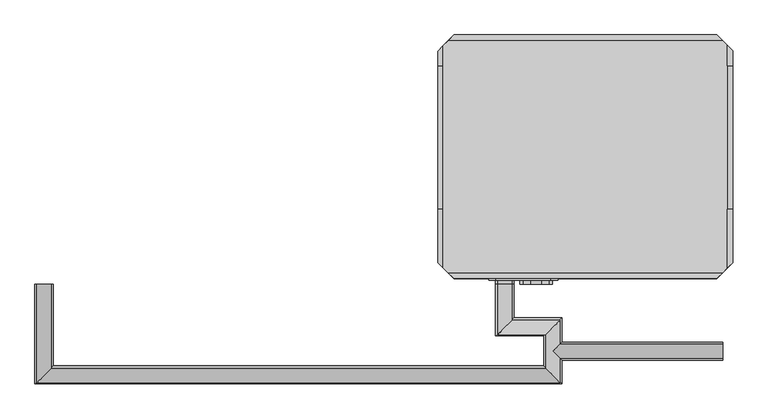
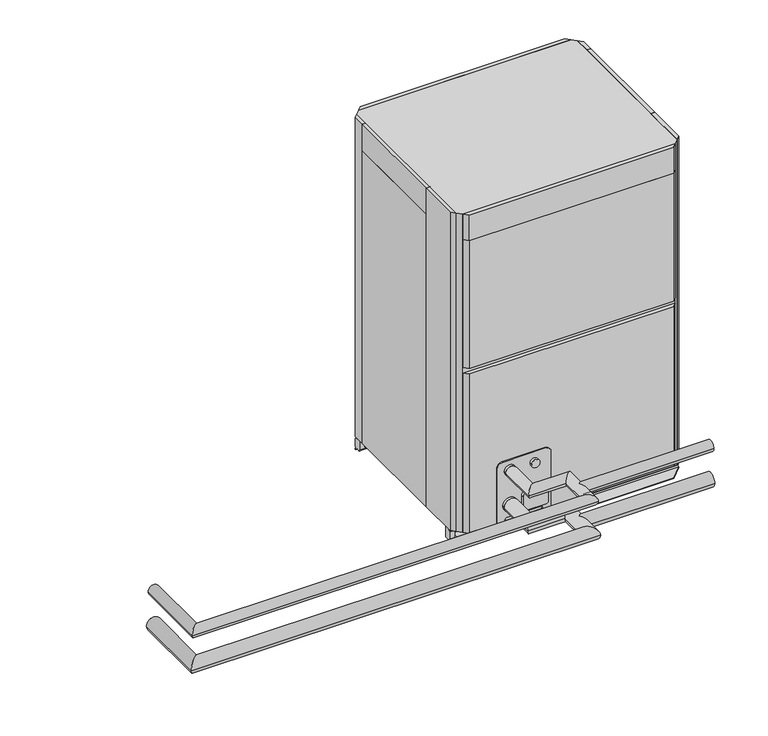
"""IFC4 building model written with IfcOpenShell, lengths in millimetres: proxy geometry, PURY-P168-288_YSJMU_Heat_Recovery_460V : PURY-P192YSJMU-A(-BS)_460V."""

from ifc_helpers import new_model, si_unit, point, frame, frame_2d, origin, place, context, project, spatial, polyline, circle_curve, ellipse_curve, trimmed, segment, composite_curve, outline, extrude, source, transform, mapped, element, save
from ifc_brep_helpers import plane_surface, cylinder_surface, revolved_surface, advanced_brep


def mechanical_equipment_f1262ded(model_context):
    return source(origin(), model_context, "Body", "SolidModel", [
        advanced_brep(
        [(-227.9552757, -397.2710787, 128.75), (-170.8052757, -397.2710787, 128.75), (-227.9552757, -709.2315266, 128.75), (-170.8052757, -652.0815266, 128.75), (1418.1947243, -709.2315266, 128.75), (1361.0447243, -652.0815266, 128.75), (1418.1947243, -635.3498061, 128.75), (1389.6197243, -606.7748061, 157.325), (1418.1947243, -578.1998061, 128.75), (1418.1947243, -502.0815266, 128.75), (1361.0447243, -559.2315266, 128.75), (1389.6197243, -606.7748061, 100.175), (1268.1947243, -502.0815266, 128.75), (1211.0447243, -559.2315266, 128.75), (1268.1947243, -397.2710787, 128.75), (1211.0447243, -397.2710787, 128.75), (1919.6197243, -635.3498061, 128.75), (1919.6197243, -578.1998061, 128.75)],
        [
            (0, 1, circle_curve(frame((-199.3802757, -397.2710787, 128.75), z_axis=(0.0, 1.0, 0.0), x_axis=(1.0, 0.0, 0.0)), 28.575)),
            (1, 0, circle_curve(frame((-199.3802757, -397.2710787, 128.75), z_axis=(0.0, 1.0, 0.0), x_axis=(1.0, 0.0, 0.0)), 28.575)),
            (0, 2),
            (2, 3, ellipse_curve(frame((-199.3802757, -680.6565266, 128.75), z_axis=(-0.7071067811865475, 0.7071067811865475, 0.0), x_axis=(0.7071067811865474, 0.7071067811865476, 0.0)), 40.4111525, 28.575)),
            (3, 1),
            (3, 2, ellipse_curve(frame((-199.3802757, -680.6565266, 128.75), z_axis=(-0.7071067811865475, 0.7071067811865475, 0.0), x_axis=(0.7071067811865474, 0.7071067811865476, 0.0)), 40.4111525, 28.575)),
            (2, 4),
            (4, 5, ellipse_curve(frame((1389.6197243, -680.6565266, 128.75), z_axis=(-0.7071067811865475, -0.7071067811865475, 0.0), x_axis=(-0.7071067811865476, 0.7071067811865474, 0.0)), 40.4111525, 28.575)),
            (5, 3),
            (5, 4, ellipse_curve(frame((1389.6197243, -680.6565266, 128.75), z_axis=(-0.7071067811865475, -0.7071067811865475, 0.0), x_axis=(-0.7071067811865476, 0.7071067811865474, 0.0)), 40.4111525, 28.575)),
            (4, 6),
            (6, 7, ellipse_curve(frame((1389.6197243, -606.7748061, 128.75), z_axis=(-0.7071067811865475, -0.7071067811865475, 0.0), x_axis=(0.7071067811865474, -0.7071067811865476, 0.0)), 40.4111525, 28.575)),
            (7, 8, ellipse_curve(frame((1389.6197243, -606.7748061, 128.75), z_axis=(-0.7071067811865475, 0.7071067811865475, 0.0), x_axis=(-0.7071067811865474, -0.7071067811865476, 0.0)), 40.4111525, 28.575)),
            (8, 9),
            (9, 10, ellipse_curve(frame((1389.6197243, -530.6565266, 128.75), z_axis=(0.7071067811865475, -0.7071067811865475, 0.0), x_axis=(-0.7071067811865474, -0.7071067811865476, 0.0)), 40.4111525, 28.575)),
            (10, 5),
            (10, 9, ellipse_curve(frame((1389.6197243, -530.6565266, 128.75), z_axis=(0.7071067811865475, -0.7071067811865475, 0.0), x_axis=(-0.7071067811865474, -0.7071067811865476, 0.0)), 40.4111525, 28.575)),
            (8, 11, ellipse_curve(frame((1389.6197243, -606.7748061, 128.75), z_axis=(-0.7071067811865475, 0.7071067811865475, 0.0), x_axis=(-0.7071067811865474, -0.7071067811865476, 0.0)), 40.4111525, 28.575)),
            (11, 6, ellipse_curve(frame((1389.6197243, -606.7748061, 128.75), z_axis=(-0.7071067811865475, -0.7071067811865475, 0.0), x_axis=(0.7071067811865474, -0.7071067811865476, 0.0)), 40.4111525, 28.575)),
            (9, 12),
            (12, 13, ellipse_curve(frame((1239.6197243, -530.6565266, 128.75), z_axis=(0.7071067811865475, -0.7071067811865475, 0.0), x_axis=(0.7071067811865476, 0.7071067811865474, 0.0)), 40.4111525, 28.575)),
            (13, 10),
            (13, 12, ellipse_curve(frame((1239.6197243, -530.6565266, 128.75), z_axis=(0.7071067811865475, -0.7071067811865475, 0.0), x_axis=(0.7071067811865476, 0.7071067811865474, 0.0)), 40.4111525, 28.575)),
            (14, 15, circle_curve(frame((1239.6197243, -397.2710787, 128.75), z_axis=(0.0, 1.0, 0.0), x_axis=(-1.0, 0.0, 0.0)), 28.575)),
            (15, 14, circle_curve(frame((1239.6197243, -397.2710787, 128.75), z_axis=(0.0, 1.0, 0.0), x_axis=(-1.0, 0.0, 0.0)), 28.575)),
            (12, 14),
            (15, 13),
            (16, 17, circle_curve(frame((1919.6197243, -606.7748061, 128.75), z_axis=(1.0, 0.0, 0.0), x_axis=(0.0, 1.0, 0.0)), 28.575)),
            (17, 16, circle_curve(frame((1919.6197243, -606.7748061, 128.75), z_axis=(1.0, 0.0, 0.0), x_axis=(0.0, 1.0, 0.0)), 28.575)),
            (17, 8),
            (6, 16),
        ],
        [
            plane_surface(frame((-199.3802757, -397.2710787, 128.75), z_axis=(0.0, 1.0, 0.0), x_axis=(0.0, 0.0, 1.0))),
            cylinder_surface(frame((-199.3802757, -397.2710787, 128.75), z_axis=(0.0, 1.0, 0.0), x_axis=(1.0, 0.0, 0.0)), 28.575),
            cylinder_surface(frame((-199.3802757, -680.6565266, 128.75), z_axis=(-1.0, 0.0, 0.0), x_axis=(0.0, 1.0, 0.0)), 28.575),
            cylinder_surface(frame((1389.6197243, -680.6565266, 128.75), z_axis=(0.0, -1.0, 0.0), x_axis=(-1.0, 0.0, 0.0)), 28.575),
            cylinder_surface(frame((1389.6197243, -530.6565266, 128.75), z_axis=(1.0, 0.0, 0.0), x_axis=(0.0, -1.0, 0.0)), 28.575),
            plane_surface(frame((1239.6197243, -397.2710787, 128.75), z_axis=(0.0, 1.0, 0.0), x_axis=(0.0, 0.0, 1.0))),
            cylinder_surface(frame((1239.6197243, -530.6565266, 128.75), z_axis=(0.0, -1.0, 0.0), x_axis=(-1.0, 0.0, 0.0)), 28.575),
            plane_surface(frame((1919.6197243, -606.7748061, 128.75), z_axis=(1.0, 0.0, 0.0), x_axis=(0.0, 0.0, 1.0))),
            cylinder_surface(frame((1389.6197243, -606.7748061, 128.75), z_axis=(-1.0, 0.0, 0.0), x_axis=(0.0, 1.0, 0.0)), 28.575),
        ],
        [
            (0, [[1, 2]]),
            (1, [[-1, 3, 4, 5]]),
            (1, [[-2, -5, 6, -3]]),
            (2, [[-4, 7, 8, 9]]),
            (2, [[-6, -9, 10, -7]]),
            (3, [[-8, 11, 12, 13, 14, 15, 16]]),
            (3, [[-10, -16, 17, -14, 18, 19, -11]]),
            (4, [[-15, 20, 21, 22]]),
            (4, [[-17, -22, 23, -20]]),
            (5, [[24, 25]]),
            (6, [[-21, 26, -25, 27]]),
            (6, [[-23, -27, -24, -26]]),
            (7, [[28, 29]]),
            (8, [[-29, 30, -13, -12, 31]]),
            (8, [[-28, -31, -19, -18, -30]]),
        ],
    ),
        advanced_brep(
        [(-221.6052757, -397.2710787, 272.67), (-177.1552757, -397.2710787, 272.67), (-221.6052757, -705.4033198, 272.67), (-177.1552757, -660.9533198, 272.67), (1411.8447243, -705.4033198, 272.67), (1367.3947243, -660.9533198, 272.67), (1411.8447243, -628.9998061, 272.67), (1389.6197243, -606.7748061, 294.895), (1411.8447243, -584.5498061, 272.67), (1411.8447243, -510.9533198, 272.67), (1367.3947243, -555.4033198, 272.67), (1389.6197243, -606.7748061, 250.445), (1261.8447243, -510.9533198, 272.67), (1217.3947243, -555.4033198, 272.67), (1261.8447243, -397.2710787, 272.67), (1217.3947243, -397.2710787, 272.67), (1919.6197243, -628.9998061, 272.67), (1919.6197243, -584.5498061, 272.67)],
        [
            (0, 1, circle_curve(frame((-199.3802757, -397.2710787, 272.67), z_axis=(0.0, 1.0, 0.0), x_axis=(1.0, 0.0, 0.0)), 22.225)),
            (1, 0, circle_curve(frame((-199.3802757, -397.2710787, 272.67), z_axis=(0.0, 1.0, 0.0), x_axis=(1.0, 0.0, 0.0)), 22.225)),
            (0, 2),
            (2, 3, ellipse_curve(frame((-199.3802757, -683.1783198, 272.67), z_axis=(-0.7071067811865475, 0.7071067811865475, 0.0), x_axis=(0.7071067811865474, 0.7071067811865476, 0.0)), 31.4308964, 22.225)),
            (3, 1),
            (3, 2, ellipse_curve(frame((-199.3802757, -683.1783198, 272.67), z_axis=(-0.7071067811865475, 0.7071067811865475, 0.0), x_axis=(0.7071067811865474, 0.7071067811865476, 0.0)), 31.4308964, 22.225)),
            (2, 4),
            (4, 5, ellipse_curve(frame((1389.6197243, -683.1783198, 272.67), z_axis=(-0.7071067811865475, -0.7071067811865475, 0.0), x_axis=(-0.7071067811865476, 0.7071067811865474, 0.0)), 31.4308964, 22.225)),
            (5, 3),
            (5, 4, ellipse_curve(frame((1389.6197243, -683.1783198, 272.67), z_axis=(-0.7071067811865475, -0.7071067811865475, 0.0), x_axis=(-0.7071067811865476, 0.7071067811865474, 0.0)), 31.4308964, 22.225)),
            (4, 6),
            (6, 7, ellipse_curve(frame((1389.6197243, -606.7748061, 272.67), z_axis=(-0.7071067811865475, -0.7071067811865475, 0.0), x_axis=(0.7071067811865474, -0.7071067811865476, 0.0)), 31.4308964, 22.225)),
            (7, 8, ellipse_curve(frame((1389.6197243, -606.7748061, 272.67), z_axis=(-0.7071067811865475, 0.7071067811865475, 0.0), x_axis=(-0.7071067811865474, -0.7071067811865476, 0.0)), 31.4308964, 22.225)),
            (8, 9),
            (9, 10, ellipse_curve(frame((1389.6197243, -533.1783198, 272.67), z_axis=(0.7071067811865475, -0.7071067811865475, 0.0), x_axis=(-0.7071067811865474, -0.7071067811865476, 0.0)), 31.4308964, 22.225)),
            (10, 5),
            (10, 9, ellipse_curve(frame((1389.6197243, -533.1783198, 272.67), z_axis=(0.7071067811865475, -0.7071067811865475, 0.0), x_axis=(-0.7071067811865474, -0.7071067811865476, 0.0)), 31.4308964, 22.225)),
            (8, 11, ellipse_curve(frame((1389.6197243, -606.7748061, 272.67), z_axis=(-0.7071067811865475, 0.7071067811865475, 0.0), x_axis=(-0.7071067811865474, -0.7071067811865476, 0.0)), 31.4308964, 22.225)),
            (11, 6, ellipse_curve(frame((1389.6197243, -606.7748061, 272.67), z_axis=(-0.7071067811865475, -0.7071067811865475, 0.0), x_axis=(0.7071067811865474, -0.7071067811865476, 0.0)), 31.4308964, 22.225)),
            (9, 12),
            (12, 13, ellipse_curve(frame((1239.6197243, -533.1783198, 272.67), z_axis=(0.7071067811865475, -0.7071067811865475, 0.0), x_axis=(0.7071067811865476, 0.7071067811865474, 0.0)), 31.4308964, 22.225)),
            (13, 10),
            (13, 12, ellipse_curve(frame((1239.6197243, -533.1783198, 272.67), z_axis=(0.7071067811865475, -0.7071067811865475, 0.0), x_axis=(0.7071067811865476, 0.7071067811865474, 0.0)), 31.4308964, 22.225)),
            (14, 15, circle_curve(frame((1239.6197243, -397.2710787, 272.67), z_axis=(0.0, 1.0, 0.0), x_axis=(-1.0, 0.0, 0.0)), 22.225)),
            (15, 14, circle_curve(frame((1239.6197243, -397.2710787, 272.67), z_axis=(0.0, 1.0, 0.0), x_axis=(-1.0, 0.0, 0.0)), 22.225)),
            (12, 14),
            (15, 13),
            (16, 17, circle_curve(frame((1919.6197243, -606.7748061, 272.67), z_axis=(1.0, 0.0, 0.0), x_axis=(0.0, 1.0, 0.0)), 22.225)),
            (17, 16, circle_curve(frame((1919.6197243, -606.7748061, 272.67), z_axis=(1.0, 0.0, 0.0), x_axis=(0.0, 1.0, 0.0)), 22.225)),
            (17, 8),
            (6, 16),
        ],
        [
            plane_surface(frame((-199.3802757, -397.2710787, 272.67), z_axis=(0.0, 1.0, 0.0), x_axis=(0.0, 0.0, 1.0))),
            cylinder_surface(frame((-199.3802757, -397.2710787, 272.67), z_axis=(0.0, 1.0, 0.0), x_axis=(1.0, 0.0, 0.0)), 22.225),
            cylinder_surface(frame((-199.3802757, -683.1783198, 272.67), z_axis=(-1.0, 0.0, 0.0), x_axis=(0.0, 1.0, 0.0)), 22.225),
            cylinder_surface(frame((1389.6197243, -683.1783198, 272.67), z_axis=(0.0, -1.0, 0.0), x_axis=(-1.0, 0.0, 0.0)), 22.225),
            cylinder_surface(frame((1389.6197243, -533.1783198, 272.67), z_axis=(1.0, 0.0, 0.0), x_axis=(0.0, -1.0, 0.0)), 22.225),
            plane_surface(frame((1239.6197243, -397.2710787, 272.67), z_axis=(0.0, 1.0, 0.0), x_axis=(0.0, 0.0, 1.0))),
            cylinder_surface(frame((1239.6197243, -533.1783198, 272.67), z_axis=(0.0, -1.0, 0.0), x_axis=(-1.0, 0.0, 0.0)), 22.225),
            plane_surface(frame((1919.6197243, -606.7748061, 272.67), z_axis=(1.0, 0.0, 0.0), x_axis=(0.0, 0.0, 1.0))),
            cylinder_surface(frame((1389.6197243, -606.7748061, 272.67), z_axis=(-1.0, 0.0, 0.0), x_axis=(0.0, 1.0, 0.0)), 22.225),
        ],
        [
            (0, [[1, 2]]),
            (1, [[-1, 3, 4, 5]]),
            (1, [[-2, -5, 6, -3]]),
            (2, [[-4, 7, 8, 9]]),
            (2, [[-6, -9, 10, -7]]),
            (3, [[-8, 11, 12, 13, 14, 15, 16]]),
            (3, [[-10, -16, 17, -14, 18, 19, -11]]),
            (4, [[-15, 20, 21, 22]]),
            (4, [[-17, -22, 23, -20]]),
            (5, [[24, 25]]),
            (6, [[-21, 26, -25, 27]]),
            (6, [[-23, -27, -24, -26]]),
            (7, [[28, 29]]),
            (8, [[-29, 30, -13, -12, 31]]),
            (8, [[-28, -31, -19, -18, -30]]),
        ],
    ),
        extrude(outline(composite_curve([segment(trimmed(circle_curve(frame_2d((148.5853631, 1296.6117511)), 9.9920268), [point((158.5773899, 1296.6117511))], [point((148.5853631, 1286.6197243))], False, "CARTESIAN"), True, "CONTINUOUS"), segment(polyline([(148.5853631, 1286.6197243), (96.5694168, 1286.6197243)]), True, "CONTINUOUS"), segment(trimmed(circle_curve(frame_2d((96.5694168, 1296.6117511)), 9.9920268), [point((96.5694168, 1286.6197243))], [point((86.5773899, 1296.6117511))], False, "CARTESIAN"), True, "CONTINUOUS"), segment(polyline([(86.5773899, 1296.6117511), (86.5773899, 1378.6276974)]), True, "CONTINUOUS"), segment(trimmed(circle_curve(frame_2d((96.5694168, 1378.6276974)), 9.9920268), [point((86.5773899, 1378.6276974))], [point((96.5694168, 1388.6197243))], False, "CARTESIAN"), True, "CONTINUOUS"), segment(polyline([(96.5694168, 1388.6197243), (148.5853631, 1388.6197243)]), True, "CONTINUOUS"), segment(trimmed(circle_curve(frame_2d((148.5853631, 1378.6276974)), 9.9920268), [point((148.5853631, 1388.6197243))], [point((158.5773899, 1378.6276974))], False, "CARTESIAN"), True, "CONTINUOUS"), segment(polyline([(158.5773899, 1378.6276974), (158.5773899, 1296.6117511)]), True, "CONTINUOUS")], self_intersect=False)), frame((0.0, -397.2710787, 0.0), z_axis=(0.0, 1.0, 0.0), x_axis=(0.0, 0.0, 1.0)), (0.0, 0.0, 1.0), 12.5),
        extrude(outline(composite_curve([segment(trimmed(circle_curve(frame_2d((292.0295314, 1383.8713302)), 21.9704686), [point((292.0295314, 1405.8417988))], [point((314.0, 1383.8713302))], False, "CARTESIAN"), True, "CONTINUOUS"), segment(polyline([(314.0, 1383.8713302), (314.0, 1212.0084686)]), True, "CONTINUOUS"), segment(trimmed(circle_curve(frame_2d((292.0295314, 1212.0084686)), 21.9704686), [point((314.0, 1212.0084686))], [point((292.0295314, 1190.038))], False, "CARTESIAN"), True, "CONTINUOUS"), segment(polyline([(292.0295314, 1190.038), (54.0, 1190.038), (54.0, 1405.8417988), (292.0295314, 1405.8417988)]), True, "CONTINUOUS")], self_intersect=False), holes=[composite_curve([segment(trimmed(circle_curve(frame_2d((66.0219765, 1364.5867184)), 7.4940201), [point((73.5159966, 1364.5867184))], [point((58.5279563, 1364.5867184))], True, "CARTESIAN"), True, "CONTINUOUS"), segment(polyline([(58.5279563, 1364.5867184), (58.5279563, 1229.6943561)]), True, "CONTINUOUS"), segment(trimmed(circle_curve(frame_2d((66.0219765, 1229.6943561)), 7.4940201), [point((58.5279563, 1229.6943561))], [point((73.5159966, 1229.6943561))], True, "CARTESIAN"), True, "CONTINUOUS"), segment(polyline([(73.5159966, 1229.6943561), (73.5159966, 1364.5867184)]), True, "CONTINUOUS")], self_intersect=False)]), frame((0.0, -384.7710787, 0.0), z_axis=(0.0, 1.0, 0.0), x_axis=(0.0, 0.0, 1.0)), (0.0, 0.0, 1.0), 4.7710787),
        extrude(outline(composite_curve([segment(trimmed(circle_curve(frame_2d((272.5206481, 1239.6197243)), 22.225), [point((272.5206481, 1217.3947243))], [point((272.5206481, 1261.8447243))], False, "CARTESIAN"), True, "CONTINUOUS"), segment(trimmed(circle_curve(frame_2d((272.5206481, 1239.6197243)), 22.225), [point((272.5206481, 1261.8447243))], [point((272.5206481, 1217.3947243))], False, "CARTESIAN"), True, "CONTINUOUS")], self_intersect=False)), frame((0.0, -397.2710787, 0.0), z_axis=(0.0, 1.0, 0.0), x_axis=(0.0, 0.0, 1.0)), (0.0, 0.0, 1.0), 12.5),
        extrude(outline(composite_curve([segment(trimmed(circle_curve(frame_2d((272.5206481, 1337.6197243)), 17.0), [point((272.5206481, 1320.6197243))], [point((272.5206481, 1354.6197243))], False, "CARTESIAN"), True, "CONTINUOUS"), segment(trimmed(circle_curve(frame_2d((272.5206481, 1337.6197243)), 17.0), [point((272.5206481, 1354.6197243))], [point((272.5206481, 1320.6197243))], False, "CARTESIAN"), True, "CONTINUOUS")], self_intersect=False)), frame((0.0, -397.2710787, 0.0), z_axis=(0.0, 1.0, 0.0), x_axis=(0.0, 0.0, 1.0)), (0.0, 0.0, 1.0), 12.5),
        extrude(outline(composite_curve([segment(trimmed(circle_curve(frame_2d((127.8409633, 1239.6197243)), 28.575), [point((127.8409633, 1211.0447243))], [point((127.8409633, 1268.1947243))], False, "CARTESIAN"), True, "CONTINUOUS"), segment(trimmed(circle_curve(frame_2d((127.8409633, 1239.6197243)), 28.575), [point((127.8409633, 1268.1947243))], [point((127.8409633, 1211.0447243))], False, "CARTESIAN"), True, "CONTINUOUS")], self_intersect=False)), frame((0.0, -397.2710787, 0.0), z_axis=(0.0, 1.0, 0.0), x_axis=(0.0, 0.0, 1.0)), (0.0, 0.0, 1.0), 12.5),
        extrude(outline(polyline([(1951.038, 284.0), (1935.038, 284.0), (1935.038, 346.9999976), (1951.038, 330.9999976), (1951.038, 284.0)])), frame((0.0, 0.0, 54.0), z_axis=(0.0, 0.0, 1.0), x_axis=(1.0, 0.0, 0.0)), (0.0, 0.0, 1.0), 1356.0),
        extrude(outline(polyline([(1935.038, -164.0), (1951.038, -164.0), (1951.038, -331.000002), (1935.038, -347.000002), (1935.038, -164.0)])), frame((0.0, 0.0, 54.0), z_axis=(0.0, 0.0, 1.0), x_axis=(1.0, 0.0, 0.0)), (0.0, 0.0, 1.0), 1356.0),
        extrude(outline(polyline([(1882.5551598, 364.0), (1882.5551598, 380.0), (1902.0379976, 380.0), (1918.0379976, 364.0), (1882.5551598, 364.0)])), frame((0.0, 0.0, 54.0), z_axis=(0.0, 0.0, 1.0), x_axis=(1.0, 0.0, 0.0)), (0.0, 0.0, 1.0), 1245.8),
        extrude(outline(polyline([(1109.870831, 380.0), (1109.870831, 364.0), (1065.4504928, 364.0), (1081.4504928, 380.0), (1109.870831, 380.0)])), frame((0.0, 0.0, 54.0), z_axis=(0.0, 0.0, 1.0), x_axis=(1.0, 0.0, 0.0)), (0.0, 0.0, 1.0), 1245.8),
        extrude(outline(polyline([(1918.0379976, 364.0), (1065.4504928, 364.0), (1081.4504928, 380.0), (1902.0379976, 380.0), (1918.0379976, 364.0)])), frame((0.0, 0.0, 1299.8), z_axis=(0.0, 0.0, 1.0), x_axis=(1.0, 0.0, 0.0)), (0.0, 0.0, 1.0), 110.2),
        extrude(outline(polyline([(1902.038002, -380.0), (1080.0379871, -380.0), (1064.0379871, -364.0), (1918.038002, -364.0), (1902.038002, -380.0)])), frame((0.0, 0.0, 1299.8), z_axis=(0.0, 0.0, 1.0), x_axis=(1.0, 0.0, 0.0)), (0.0, 0.0, 1.0), 110.2),
        extrude(outline(polyline([(1064.0379871, -364.0), (1918.038002, -364.0), (1902.038002, -380.0), (1080.0379871, -380.0), (1064.0379871, -364.0)])), frame((0.0, 0.0, 755.5000076), z_axis=(0.0, 0.0, 1.0), x_axis=(1.0, 0.0, 0.0)), (0.0, 0.0, 1.0), 544.2999924),
        extrude(outline(polyline([(1047.038, -347.0000129), (1047.038, 345.5875072), (1065.4504928, 364.0), (1918.0379976, 364.0), (1935.038, 346.9999976), (1935.038, -347.000002), (1918.038002, -364.0), (1064.0379871, -364.0), (1047.038, -347.0000129)])), frame((0.0, 0.0, 54.0), z_axis=(0.0, 0.0, 1.0), x_axis=(1.0, 0.0, 0.0)), (0.0, 0.0, 1.0), 1356.0),
        extrude(outline(polyline([(1047.038, 284.0), (1031.038, 284.0), (1031.038, 329.5875072), (1047.038, 345.5875072), (1047.038, 284.0)])), frame((0.0, 0.0, 54.0), z_axis=(0.0, 0.0, 1.0), x_axis=(1.0, 0.0, 0.0)), (0.0, 0.0, 1.0), 1356.0),
        extrude(outline(polyline([(1031.038, -164.0), (1047.038, -164.0), (1047.038, -347.0000129), (1031.038, -331.0000129), (1031.038, -164.0)])), frame((0.0, 0.0, 54.0), z_axis=(0.0, 0.0, 1.0), x_axis=(1.0, 0.0, 0.0)), (0.0, 0.0, 1.0), 1356.0),
        extrude(outline(polyline([(1064.0379871, -364.0), (1918.038002, -364.0), (1902.038002, -380.0), (1080.0379871, -380.0), (1064.0379871, -364.0)])), frame((0.0, 0.0, 54.0), z_axis=(0.0, 0.0, 1.0), x_axis=(1.0, 0.0, 0.0)), (0.0, 0.0, 1.0), 678.5000074),
        extrude(outline(polyline([(1491.038, 364.0), (1491.038, 380.0), (1882.5551598, 380.0), (1882.5551598, 364.0), (1491.038, 364.0)])), frame((0.0, 0.0, 54.0), z_axis=(0.0, 0.0, 1.0), x_axis=(1.0, 0.0, 0.0)), (0.0, 0.0, 1.0), 1245.8),
        extrude(outline(polyline([(1109.870831, 364.0), (1109.870831, 380.0), (1491.038, 380.0), (1491.038, 364.0), (1109.870831, 364.0)])), frame((0.0, 0.0, 54.0), z_axis=(0.0, 0.0, 1.0), x_axis=(1.0, 0.0, 0.0)), (0.0, 0.0, 1.0), 1245.8),
        advanced_brep(
        [(1951.038, 330.9999976, 2.3), (1951.038, 330.9999976, 0.0), (1902.0379976, 380.0, 0.0), (1902.0379976, 380.0, 2.3), (1031.038, 329.5875072, 0.0), (1031.038, 329.5875072, 2.3), (1081.4504928, 380.0, 2.3), (1081.4504928, 380.0, 0.0), (1951.038, 329.5875072, 2.3), (1951.038, 324.5875071, 7.3000001), (1951.038, 324.5875071, 11.7000001), (1951.038, 325.5875071, 12.7000001), (1951.038, 327.5875072, 12.7000001), (1951.038, 327.5875072, 47.3000005), (1951.038, 325.5875071, 47.3000005), (1951.038, 324.5875071, 48.3000005), (1951.038, 324.5875071, 50.0000004), (1951.038, 320.5875077, 53.9999997), (1951.038, 299.5875069, 53.9999997), (1951.038, 299.5875069, 14.0000001), (1951.038, 304.5875069, 9.0000001), (1951.038, 322.2875071, 9.0000001), (1951.038, 322.2875071, 7.3000001), (1951.038, 329.5875072, 0.0), (1031.038, 322.2875071, 7.3000001), (1031.038, 322.2875071, 9.0000001), (1031.038, 304.5875069, 9.0000001), (1031.038, 299.5875069, 14.0000001), (1031.038, 299.5875069, 53.9999997), (1031.038, 320.5875077, 53.9999997), (1031.038, 324.5875071, 50.0000004), (1031.038, 324.5875071, 48.3000005), (1031.038, 325.5875071, 47.3000005), (1031.038, 327.5875072, 47.3000005), (1031.038, 327.5875072, 12.7000001), (1031.038, 325.5875071, 12.7000001), (1031.038, 324.5875071, 11.7000001), (1031.038, 324.5875071, 7.3000001), (1922.288009, 327.5875072, 45.0000005), (1880.7880086, 327.5875072, 45.0000005), (1874.7880085, 327.5875072, 39.0000004), (1874.7880085, 327.5875072, 21.0000002), (1880.7880086, 327.5875072, 15.0000002), (1922.288009, 327.5875072, 15.0000002), (1928.2880091, 327.5875072, 21.0000002), (1928.2880091, 327.5875072, 39.0000004), (1059.0380003, 327.5875072, 45.0000005), (1053.0380002, 327.5875072, 39.0000004), (1053.0380002, 327.5875072, 21.0000002), (1059.0380003, 327.5875072, 15.0000002), (1100.5380007, 327.5875072, 15.0000002), (1106.5380008, 327.5875072, 21.0000002), (1106.5380008, 327.5875072, 39.0000004), (1100.5380007, 327.5875072, 45.0000005), (1880.7880086, 299.5875069, 45.0000005), (1922.288009, 299.5875069, 45.0000005), (1928.2880091, 299.5875069, 39.0000004), (1928.2880091, 299.5875069, 21.0000002), (1922.288009, 299.5875069, 15.0000002), (1880.7880086, 299.5875069, 15.0000002), (1874.7880085, 299.5875069, 21.0000002), (1874.7880085, 299.5875069, 39.0000004), (1053.0380002, 299.5875069, 39.0000004), (1059.0380003, 299.5875069, 45.0000005), (1100.5380007, 299.5875069, 45.0000005), (1106.5380008, 299.5875069, 39.0000004), (1106.5380008, 299.5875069, 21.0000002), (1100.5380007, 299.5875069, 15.0000002), (1059.0380003, 299.5875069, 15.0000002), (1053.0380002, 299.5875069, 21.0000002)],
        [
            (0, 1),
            (1, 2),
            (2, 3),
            (3, 0),
            (4, 5),
            (5, 6),
            (6, 7),
            (7, 4),
            (8, 9, circle_curve(frame((1951.038, 329.5875072, 7.3000001), z_axis=(-1.0, 0.0, 0.0), x_axis=(0.0, 1.0, 0.0)), 5.0000001)),
            (9, 10),
            (10, 11, circle_curve(frame((1951.038, 325.5875071, 11.7000001), z_axis=(-1.0, 0.0, 0.0), x_axis=(0.0, 1.0, 0.0)), 1.0)),
            (11, 12),
            (12, 13),
            (13, 14),
            (14, 15, circle_curve(frame((1951.038, 325.5875071, 48.3000005), z_axis=(-1.0, 0.0, 0.0), x_axis=(0.0, 1.0, 0.0)), 1.0)),
            (15, 16),
            (16, 17, circle_curve(frame((1951.038, 320.5875077, 50.0000004), z_axis=(1.0, 0.0, 0.0), x_axis=(0.0, 1.0, 0.0)), 3.9999994)),
            (17, 18),
            (18, 19),
            (19, 20, circle_curve(frame((1951.038, 304.5875069, 14.0000001), z_axis=(1.0, 0.0, 0.0), x_axis=(0.0, 1.0, 0.0)), 5.0000001)),
            (20, 21),
            (21, 22),
            (22, 23, circle_curve(frame((1951.038, 329.5875072, 7.3000001), z_axis=(1.0, 0.0, 0.0), x_axis=(0.0, 1.0, 0.0)), 7.3000001)),
            (23, 1),
            (0, 8),
            (4, 24, circle_curve(frame((1031.038, 329.5875072, 7.3000001), z_axis=(-1.0, 0.0, 0.0), x_axis=(0.0, 1.0, 0.0)), 7.3000001)),
            (24, 25),
            (25, 26),
            (26, 27, circle_curve(frame((1031.038, 304.5875069, 14.0000001), z_axis=(-1.0, 0.0, 0.0), x_axis=(0.0, 1.0, 0.0)), 5.0000001)),
            (27, 28),
            (28, 29),
            (29, 30, circle_curve(frame((1031.038, 320.5875077, 50.0000004), z_axis=(-1.0, 0.0, 0.0), x_axis=(0.0, 1.0, 0.0)), 3.9999994)),
            (30, 31),
            (31, 32, circle_curve(frame((1031.038, 325.5875071, 48.3000005), z_axis=(1.0, 0.0, 0.0), x_axis=(0.0, 1.0, 0.0)), 1.0)),
            (32, 33),
            (33, 34),
            (34, 35),
            (35, 36, circle_curve(frame((1031.038, 325.5875071, 11.7000001), z_axis=(1.0, 0.0, 0.0), x_axis=(0.0, 1.0, 0.0)), 1.0)),
            (36, 37),
            (37, 5, circle_curve(frame((1031.038, 329.5875072, 7.3000001), z_axis=(1.0, 0.0, 0.0), x_axis=(0.0, 1.0, 0.0)), 5.0000001)),
            (8, 5),
            (37, 9),
            (36, 10),
            (35, 11),
            (34, 12),
            (33, 13),
            (38, 39),
            (39, 40, circle_curve(frame((1880.7880086, 327.5875072, 39.0000004), z_axis=(0.0, -1.0, 0.0), x_axis=(1.0, 0.0, 0.0)), 6.0000001)),
            (40, 41),
            (41, 42, circle_curve(frame((1880.7880086, 327.5875072, 21.0000002), z_axis=(0.0, -1.0, 0.0), x_axis=(1.0, 0.0, 0.0)), 6.0000001)),
            (42, 43),
            (43, 44, circle_curve(frame((1922.288009, 327.5875072, 21.0000002), z_axis=(0.0, -1.0, 0.0), x_axis=(1.0, 0.0, 0.0)), 6.0000001)),
            (44, 45),
            (45, 38, circle_curve(frame((1922.288009, 327.5875072, 39.0000004), z_axis=(0.0, -1.0, 0.0), x_axis=(1.0, 0.0, 0.0)), 6.0000001)),
            (46, 47, circle_curve(frame((1059.0380003, 327.5875072, 39.0000004), z_axis=(0.0, -1.0, 0.0), x_axis=(1.0, 0.0, 0.0)), 6.0000001)),
            (47, 48),
            (48, 49, circle_curve(frame((1059.0380003, 327.5875072, 21.0000002), z_axis=(0.0, -1.0, 0.0), x_axis=(1.0, 0.0, 0.0)), 6.0000001)),
            (49, 50),
            (50, 51, circle_curve(frame((1100.5380007, 327.5875072, 21.0000002), z_axis=(0.0, -1.0, 0.0), x_axis=(1.0, 0.0, 0.0)), 6.0000001)),
            (51, 52),
            (52, 53, circle_curve(frame((1100.5380007, 327.5875072, 39.0000004), z_axis=(0.0, -1.0, 0.0), x_axis=(1.0, 0.0, 0.0)), 6.0000001)),
            (53, 46),
            (32, 14),
            (31, 15),
            (30, 16),
            (29, 17),
            (28, 18),
            (27, 19),
            (54, 55),
            (55, 56, circle_curve(frame((1922.288009, 299.5875069, 39.0000004), z_axis=(0.0, 1.0, 0.0), x_axis=(1.0, 0.0, 0.0)), 6.0000001)),
            (56, 57),
            (57, 58, circle_curve(frame((1922.288009, 299.5875069, 21.0000002), z_axis=(0.0, 1.0, 0.0), x_axis=(1.0, 0.0, 0.0)), 6.0000001)),
            (58, 59),
            (59, 60, circle_curve(frame((1880.7880086, 299.5875069, 21.0000002), z_axis=(0.0, 1.0, 0.0), x_axis=(1.0, 0.0, 0.0)), 6.0000001)),
            (60, 61),
            (61, 54, circle_curve(frame((1880.7880086, 299.5875069, 39.0000004), z_axis=(0.0, 1.0, 0.0), x_axis=(1.0, 0.0, 0.0)), 6.0000001)),
            (62, 63, circle_curve(frame((1059.0380003, 299.5875069, 39.0000004), z_axis=(0.0, 1.0, 0.0), x_axis=(1.0, 0.0, 0.0)), 6.0000001)),
            (63, 64),
            (64, 65, circle_curve(frame((1100.5380007, 299.5875069, 39.0000004), z_axis=(0.0, 1.0, 0.0), x_axis=(1.0, 0.0, 0.0)), 6.0000001)),
            (65, 66),
            (66, 67, circle_curve(frame((1100.5380007, 299.5875069, 21.0000002), z_axis=(0.0, 1.0, 0.0), x_axis=(1.0, 0.0, 0.0)), 6.0000001)),
            (67, 68),
            (68, 69, circle_curve(frame((1059.0380003, 299.5875069, 21.0000002), z_axis=(0.0, 1.0, 0.0), x_axis=(1.0, 0.0, 0.0)), 6.0000001)),
            (69, 62),
            (26, 20),
            (25, 21),
            (24, 22),
            (4, 23),
            (7, 2),
            (6, 3),
            (38, 55),
            (54, 39),
            (61, 40),
            (60, 41),
            (59, 42),
            (58, 43),
            (57, 44),
            (56, 45),
            (46, 63),
            (62, 47),
            (69, 48),
            (68, 49),
            (67, 50),
            (66, 51),
            (65, 52),
            (64, 53),
        ],
        [
            plane_surface(frame((1902.0379976, 380.0, 1410.0), z_axis=(0.7071067811865485, 0.7071067811865466, 0.0), x_axis=(0.0, 0.0, -1.0))),
            plane_surface(frame((1031.038, 329.5875072, 1410.0), z_axis=(-0.7071067811865466, 0.7071067811865485, 0.0), x_axis=(0.0, 0.0, -1.0))),
            plane_surface(frame((1951.038, 334.5875072, 7.3000001), z_axis=(1.0, 0.0, 0.0), x_axis=(0.0, 0.0, -1.0))),
            plane_surface(frame((1031.038, 334.5875072, 7.3000001), z_axis=(-1.0, 0.0, 0.0), x_axis=(0.0, 0.0, 1.0))),
            revolved_surface(polyline([(1031.038, 334.5875073, 7.3000001), (1951.038, 334.5875073, 7.3000001)]), (1031.038, 329.5875072, 7.3000001), (-1.0, 0.0, 0.0)),
            plane_surface(frame((1951.038, 324.5875071, 7.3000001), z_axis=(0.0, 1.0, 0.0), x_axis=(-1.0, 0.0, 0.0))),
            revolved_surface(polyline([(1031.038, 326.5875071, 11.7000001), (1951.038, 326.5875071, 11.7000001)]), (1031.038, 325.5875071, 11.7000001), (-1.0, 0.0, 0.0)),
            plane_surface(frame((1951.038, 325.5875071, 12.7000001), z_axis=(0.0, 0.0, -1.0), x_axis=(-1.0, 0.0, 0.0))),
            plane_surface(frame((1951.038, 327.5875072, 12.7000001), z_axis=(0.0, 1.0, 0.0), x_axis=(-1.0, 0.0, 0.0))),
            plane_surface(frame((1951.038, 327.5875072, 47.3000005), z_axis=(0.0, 0.0, 1.0), x_axis=(-1.0, 0.0, 0.0))),
            revolved_surface(polyline([(1031.038, 326.5875071, 48.3000005), (1951.038, 326.5875071, 48.3000005)]), (1031.038, 325.5875071, 48.3000005), (-1.0, 0.0, 0.0)),
            plane_surface(frame((1951.038, 324.5875071, 48.3000005), z_axis=(0.0, 1.0, 0.0), x_axis=(-1.0, 0.0, 0.0))),
            cylinder_surface(frame((1031.038, 320.5875077, 50.0000004), z_axis=(1.0, 0.0, 0.0), x_axis=(0.0, 1.0, 0.0)), 3.9999994),
            plane_surface(frame((1951.038, 320.5875077, 53.9999997), z_axis=(0.0, 0.0, 1.0), x_axis=(-1.0, 0.0, 0.0))),
            plane_surface(frame((1951.038, 299.5875069, 53.9999997), z_axis=(0.0, -1.0, 0.0), x_axis=(-1.0, 0.0, 0.0))),
            cylinder_surface(frame((1031.038, 304.5875069, 14.0000001), z_axis=(1.0, 0.0, 0.0), x_axis=(0.0, 1.0, 0.0)), 5.0000001),
            plane_surface(frame((1951.038, 304.5875069, 9.0000001), z_axis=(0.0, 0.0, -1.0), x_axis=(-1.0, 0.0, 0.0))),
            plane_surface(frame((1951.038, 322.2875071, 9.0000001), z_axis=(0.0, -1.0, 0.0), x_axis=(-1.0, 0.0, 0.0))),
            cylinder_surface(frame((1031.038, 329.5875072, 7.3000001), z_axis=(1.0, 0.0, 0.0), x_axis=(0.0, 1.0, 0.0)), 7.3000001),
            plane_surface(frame((1951.038, 329.5875072, 0.0), z_axis=(0.0, 0.0, -1.0), x_axis=(-1.0, 0.0, 0.0))),
            plane_surface(frame((1951.038, 380.0, 0.0), z_axis=(0.0, 1.0, 0.0), x_axis=(-1.0, 0.0, 0.0))),
            plane_surface(frame((1951.038, 380.0, 2.3), z_axis=(0.0, 0.0, 1.0), x_axis=(-1.0, 0.0, 0.0))),
            plane_surface(frame((1922.288009, -339.0, 45.0000005), z_axis=(0.0, 0.0, -1.0), x_axis=(0.0, 1.0, 0.0))),
            revolved_surface(polyline([(1886.7880087, 299.5875069, 39.0000004), (1886.7880087, 327.5875072, 39.0000004)]), (1880.7880086, 339.0, 39.0000004), (0.0, -1.0, 0.0)),
            plane_surface(frame((1874.7880085, -339.0, 39.0000004), z_axis=(1.0, 0.0, 0.0), x_axis=(0.0, 1.0, 0.0))),
            revolved_surface(polyline([(1886.7880087, 299.5875069, 21.0000002), (1886.7880087, 327.5875072, 21.0000002)]), (1880.7880086, 339.0, 21.0000002), (0.0, -1.0, 0.0)),
            plane_surface(frame((1880.7880086, -339.0, 15.0000002), z_axis=(0.0, 0.0, 1.0), x_axis=(0.0, 1.0, 0.0))),
            revolved_surface(polyline([(1928.2880091000002, 299.5875069, 21.0000002), (1928.2880091000002, 327.5875072, 21.0000002)]), (1922.288009, 339.0, 21.0000002), (0.0, -1.0, 0.0)),
            plane_surface(frame((1928.2880091, -339.0, 21.0000002), z_axis=(-1.0, 0.0, 0.0), x_axis=(0.0, 1.0, 0.0))),
            revolved_surface(polyline([(1928.2880091000002, 299.5875069, 39.0000004), (1928.2880091000002, 327.5875072, 39.0000004)]), (1922.288009, 339.0, 39.0000004), (0.0, -1.0, 0.0)),
            revolved_surface(polyline([(1065.0380004, 299.5875069, 39.0000004), (1065.0380004, 327.5875072, 39.0000004)]), (1059.0380003, 0.0, 39.0000004), (0.0, -1.0, 0.0)),
            plane_surface(frame((1053.0380002, -339.0, 39.0000004), z_axis=(1.0, 0.0, 0.0), x_axis=(0.0, 1.0, 0.0))),
            revolved_surface(polyline([(1065.0380004, 299.5875069, 21.0000002), (1065.0380004, 327.5875072, 21.0000002)]), (1059.0380003, 0.0, 21.0000002), (0.0, -1.0, 0.0)),
            plane_surface(frame((1059.0380003, -339.0, 15.0000002), z_axis=(0.0, 0.0, 1.0), x_axis=(0.0, 1.0, 0.0))),
            revolved_surface(polyline([(1106.5380008000002, 299.5875069, 21.0000002), (1106.5380008000002, 327.5875072, 21.0000002)]), (1100.5380007, 0.0, 21.0000002), (0.0, -1.0, 0.0)),
            plane_surface(frame((1106.5380008, -339.0, 21.0000002), z_axis=(-1.0, 0.0, 0.0), x_axis=(0.0, 1.0, 0.0))),
            revolved_surface(polyline([(1106.5380008000002, 299.5875069, 39.0000004), (1106.5380008000002, 327.5875072, 39.0000004)]), (1100.5380007, 0.0, 39.0000004), (0.0, -1.0, 0.0)),
            plane_surface(frame((1100.5380007, -339.0, 45.0000005), z_axis=(0.0, 0.0, -1.0), x_axis=(0.0, 1.0, 0.0))),
        ],
        [
            (0, [[1, 2, 3, 4]]),
            (1, [[5, 6, 7, 8]]),
            (2, [[9, 10, 11, 12, 13, 14, 15, 16, 17, 18, 19, 20, 21, 22, 23, 24, -1, 25]]),
            (3, [[26, 27, 28, 29, 30, 31, 32, 33, 34, 35, 36, 37, 38, 39, 40, -5]]),
            (4, [[-9, 41, -40, 42]]),
            (5, [[-10, -42, -39, 43]]),
            (6, [[-11, -43, -38, 44]]),
            (7, [[-12, -44, -37, 45]]),
            (8, [[-13, -45, -36, 46], [47, 48, 49, 50, 51, 52, 53, 54], [55, 56, 57, 58, 59, 60, 61, 62]]),
            (9, [[-14, -46, -35, 63]]),
            (10, [[-15, -63, -34, 64]]),
            (11, [[-16, -64, -33, 65]]),
            (12, [[-17, -65, -32, 66]]),
            (13, [[-18, -66, -31, 67]]),
            (14, [[-19, -67, -30, 68], [69, 70, 71, 72, 73, 74, 75, 76], [77, 78, 79, 80, 81, 82, 83, 84]]),
            (15, [[-20, -68, -29, 85]]),
            (16, [[-21, -85, -28, 86]]),
            (17, [[-22, -86, -27, 87]]),
            (18, [[-23, -87, -26, 88]]),
            (19, [[-88, -8, 89, -2, -24]]),
            (20, [[-89, -7, 90, -3]]),
            (21, [[-41, -25, -4, -90, -6]]),
            (22, [[91, -69, 92, -47]]),
            (23, [[-92, -76, 93, -48]]),
            (24, [[-93, -75, 94, -49]]),
            (25, [[-94, -74, 95, -50]]),
            (26, [[-95, -73, 96, -51]]),
            (27, [[-96, -72, 97, -52]]),
            (28, [[-97, -71, 98, -53]]),
            (29, [[-91, -54, -98, -70]]),
            (30, [[99, -77, 100, -55]]),
            (31, [[-100, -84, 101, -56]]),
            (32, [[-101, -83, 102, -57]]),
            (33, [[-102, -82, 103, -58]]),
            (34, [[-103, -81, 104, -59]]),
            (35, [[-104, -80, 105, -60]]),
            (36, [[-105, -79, 106, -61]]),
            (37, [[-99, -62, -106, -78]]),
        ],
    ),
        advanced_brep(
        [(1951.038, -331.000002, 0.0), (1951.038, -331.000002, 2.3), (1902.038002, -380.0, 2.3), (1902.038002, -380.0, 0.0), (1031.038, -331.0000129, 2.3), (1031.038, -331.0000129, 0.0), (1080.0379871, -380.0, 0.0), (1080.0379871, -380.0, 2.3), (1951.038, -329.9000072, 0.0), (1951.038, -322.6000071, 7.3000001), (1951.038, -322.6000071, 9.0000001), (1951.038, -304.9000069, 9.0000001), (1951.038, -299.9000069, 14.0000001), (1951.038, -299.9000069, 53.9999997), (1951.038, -320.9000077, 53.9999997), (1951.038, -324.9000071, 50.0000004), (1951.038, -324.9000071, 48.3000005), (1951.038, -325.9000071, 47.3000005), (1951.038, -327.9000072, 47.3000005), (1951.038, -327.9000072, 12.7000001), (1951.038, -325.9000071, 12.7000001), (1951.038, -324.9000071, 11.7000001), (1951.038, -324.9000071, 7.3000001), (1951.038, -329.9000072, 2.3), (1031.038, -329.9000072, 2.3), (1031.038, -324.9000071, 7.3000001), (1031.038, -324.9000071, 11.7000001), (1031.038, -325.9000071, 12.7000001), (1031.038, -327.9000072, 12.7000001), (1031.038, -327.9000072, 47.3000005), (1031.038, -325.9000071, 47.3000005), (1031.038, -324.9000071, 48.3000005), (1031.038, -324.9000071, 50.0000004), (1031.038, -320.9000077, 53.9999997), (1031.038, -299.9000069, 53.9999997), (1031.038, -299.9000069, 14.0000001), (1031.038, -304.9000069, 9.0000001), (1031.038, -322.6000071, 9.0000001), (1031.038, -322.6000071, 7.3000001), (1031.038, -329.9000072, 0.0), (1922.288009, -299.9000069, 45.0000005), (1880.7880086, -299.9000069, 45.0000005), (1874.7880085, -299.9000069, 39.0000004), (1874.7880085, -299.9000069, 21.0000002), (1880.7880086, -299.9000069, 15.0000002), (1922.288009, -299.9000069, 15.0000002), (1928.2880091, -299.9000069, 21.0000002), (1928.2880091, -299.9000069, 39.0000004), (1059.0380003, -299.9000069, 45.0000005), (1053.0380002, -299.9000069, 39.0000004), (1053.0380002, -299.9000069, 21.0000002), (1059.0380003, -299.9000069, 15.0000002), (1100.5380007, -299.9000069, 15.0000002), (1106.5380008, -299.9000069, 21.0000002), (1106.5380008, -299.9000069, 39.0000004), (1100.5380007, -299.9000069, 45.0000005), (1880.7880086, -327.9000072, 45.0000005), (1922.288009, -327.9000072, 45.0000005), (1928.2880091, -327.9000072, 39.0000004), (1928.2880091, -327.9000072, 21.0000002), (1922.288009, -327.9000072, 15.0000002), (1880.7880086, -327.9000072, 15.0000002), (1874.7880085, -327.9000072, 21.0000002), (1874.7880085, -327.9000072, 39.0000004), (1053.0380002, -327.9000072, 39.0000004), (1059.0380003, -327.9000072, 45.0000005), (1100.5380007, -327.9000072, 45.0000005), (1106.5380008, -327.9000072, 39.0000004), (1106.5380008, -327.9000072, 21.0000002), (1100.5380007, -327.9000072, 15.0000002), (1059.0380003, -327.9000072, 15.0000002), (1053.0380002, -327.9000072, 21.0000002)],
        [
            (0, 1),
            (1, 2),
            (2, 3),
            (3, 0),
            (4, 5),
            (5, 6),
            (6, 7),
            (7, 4),
            (8, 9, circle_curve(frame((1951.038, -329.9000072, 7.3000001), z_axis=(1.0, 0.0, 0.0), x_axis=(0.0, 1.0, 0.0)), 7.3000001)),
            (9, 10),
            (10, 11),
            (11, 12, circle_curve(frame((1951.038, -304.9000069, 14.0000001), z_axis=(1.0, 0.0, 0.0), x_axis=(0.0, 1.0, 0.0)), 5.0000001)),
            (12, 13),
            (13, 14),
            (14, 15, circle_curve(frame((1951.038, -320.9000077, 50.0000004), z_axis=(1.0, 0.0, 0.0), x_axis=(0.0, 1.0, 0.0)), 3.9999994)),
            (15, 16),
            (16, 17, circle_curve(frame((1951.038, -325.9000071, 48.3000005), z_axis=(-1.0, 0.0, 0.0), x_axis=(0.0, 1.0, 0.0)), 1.0)),
            (17, 18),
            (18, 19),
            (19, 20),
            (20, 21, circle_curve(frame((1951.038, -325.9000071, 11.7000001), z_axis=(-1.0, 0.0, 0.0), x_axis=(0.0, 1.0, 0.0)), 1.0)),
            (21, 22),
            (22, 23, circle_curve(frame((1951.038, -329.9000072, 7.3000001), z_axis=(-1.0, 0.0, 0.0), x_axis=(0.0, 1.0, 0.0)), 5.0000001)),
            (23, 1),
            (0, 8),
            (24, 25, circle_curve(frame((1031.038, -329.9000072, 7.3000001), z_axis=(1.0, 0.0, 0.0), x_axis=(0.0, 1.0, 0.0)), 5.0000001)),
            (25, 26),
            (26, 27, circle_curve(frame((1031.038, -325.9000071, 11.7000001), z_axis=(1.0, 0.0, 0.0), x_axis=(0.0, 1.0, 0.0)), 1.0)),
            (27, 28),
            (28, 29),
            (29, 30),
            (30, 31, circle_curve(frame((1031.038, -325.9000071, 48.3000005), z_axis=(1.0, 0.0, 0.0), x_axis=(0.0, 1.0, 0.0)), 1.0)),
            (31, 32),
            (32, 33, circle_curve(frame((1031.038, -320.9000077, 50.0000004), z_axis=(-1.0, 0.0, 0.0), x_axis=(0.0, 1.0, 0.0)), 3.9999994)),
            (33, 34),
            (34, 35),
            (35, 36, circle_curve(frame((1031.038, -304.9000069, 14.0000001), z_axis=(-1.0, 0.0, 0.0), x_axis=(0.0, 1.0, 0.0)), 5.0000001)),
            (36, 37),
            (37, 38),
            (38, 39, circle_curve(frame((1031.038, -329.9000072, 7.3000001), z_axis=(-1.0, 0.0, 0.0), x_axis=(0.0, 1.0, 0.0)), 7.3000001)),
            (39, 5),
            (4, 24),
            (23, 24),
            (7, 2),
            (6, 3),
            (39, 8),
            (38, 9),
            (37, 10),
            (36, 11),
            (35, 12),
            (34, 13),
            (40, 41),
            (41, 42, circle_curve(frame((1880.7880086, -299.9000069, 39.0000004), z_axis=(0.0, -1.0, 0.0), x_axis=(1.0, 0.0, 0.0)), 6.0000001)),
            (42, 43),
            (43, 44, circle_curve(frame((1880.7880086, -299.9000069, 21.0000002), z_axis=(0.0, -1.0, 0.0), x_axis=(1.0, 0.0, 0.0)), 6.0000001)),
            (44, 45),
            (45, 46, circle_curve(frame((1922.288009, -299.9000069, 21.0000002), z_axis=(0.0, -1.0, 0.0), x_axis=(1.0, 0.0, 0.0)), 6.0000001)),
            (46, 47),
            (47, 40, circle_curve(frame((1922.288009, -299.9000069, 39.0000004), z_axis=(0.0, -1.0, 0.0), x_axis=(1.0, 0.0, 0.0)), 6.0000001)),
            (48, 49, circle_curve(frame((1059.0380003, -299.9000069, 39.0000004), z_axis=(0.0, -1.0, 0.0), x_axis=(1.0, 0.0, 0.0)), 6.0000001)),
            (49, 50),
            (50, 51, circle_curve(frame((1059.0380003, -299.9000069, 21.0000002), z_axis=(0.0, -1.0, 0.0), x_axis=(1.0, 0.0, 0.0)), 6.0000001)),
            (51, 52),
            (52, 53, circle_curve(frame((1100.5380007, -299.9000069, 21.0000002), z_axis=(0.0, -1.0, 0.0), x_axis=(1.0, 0.0, 0.0)), 6.0000001)),
            (53, 54),
            (54, 55, circle_curve(frame((1100.5380007, -299.9000069, 39.0000004), z_axis=(0.0, -1.0, 0.0), x_axis=(1.0, 0.0, 0.0)), 6.0000001)),
            (55, 48),
            (33, 14),
            (32, 15),
            (31, 16),
            (30, 17),
            (29, 18),
            (28, 19),
            (56, 57),
            (57, 58, circle_curve(frame((1922.288009, -327.9000072, 39.0000004), z_axis=(0.0, 1.0, 0.0), x_axis=(1.0, 0.0, 0.0)), 6.0000001)),
            (58, 59),
            (59, 60, circle_curve(frame((1922.288009, -327.9000072, 21.0000002), z_axis=(0.0, 1.0, 0.0), x_axis=(1.0, 0.0, 0.0)), 6.0000001)),
            (60, 61),
            (61, 62, circle_curve(frame((1880.7880086, -327.9000072, 21.0000002), z_axis=(0.0, 1.0, 0.0), x_axis=(1.0, 0.0, 0.0)), 6.0000001)),
            (62, 63),
            (63, 56, circle_curve(frame((1880.7880086, -327.9000072, 39.0000004), z_axis=(0.0, 1.0, 0.0), x_axis=(1.0, 0.0, 0.0)), 6.0000001)),
            (64, 65, circle_curve(frame((1059.0380003, -327.9000072, 39.0000004), z_axis=(0.0, 1.0, 0.0), x_axis=(1.0, 0.0, 0.0)), 6.0000001)),
            (65, 66),
            (66, 67, circle_curve(frame((1100.5380007, -327.9000072, 39.0000004), z_axis=(0.0, 1.0, 0.0), x_axis=(1.0, 0.0, 0.0)), 6.0000001)),
            (67, 68),
            (68, 69, circle_curve(frame((1100.5380007, -327.9000072, 21.0000002), z_axis=(0.0, 1.0, 0.0), x_axis=(1.0, 0.0, 0.0)), 6.0000001)),
            (69, 70),
            (70, 71, circle_curve(frame((1059.0380003, -327.9000072, 21.0000002), z_axis=(0.0, 1.0, 0.0), x_axis=(1.0, 0.0, 0.0)), 6.0000001)),
            (71, 64),
            (27, 20),
            (26, 21),
            (25, 22),
            (40, 57),
            (56, 41),
            (63, 42),
            (62, 43),
            (61, 44),
            (60, 45),
            (59, 46),
            (58, 47),
            (48, 65),
            (64, 49),
            (71, 50),
            (70, 51),
            (69, 52),
            (68, 53),
            (67, 54),
            (66, 55),
        ],
        [
            plane_surface(frame((1951.038, -331.000002, 1410.0), z_axis=(0.707106781186548, -0.707106781186547, 0.0), x_axis=(0.0, 0.0, -1.0))),
            plane_surface(frame((1080.0379871, -380.0, 1410.0), z_axis=(-0.7071067811865486, -0.7071067811865466, 0.0), x_axis=(0.0, 0.0, -1.0))),
            plane_surface(frame((1951.038, 334.5875072, 7.3000001), z_axis=(1.0, 0.0, 0.0), x_axis=(0.0, 0.0, -1.0))),
            plane_surface(frame((1031.038, 334.5875072, 7.3000001), z_axis=(-1.0, 0.0, 0.0), x_axis=(0.0, 0.0, 1.0))),
            plane_surface(frame((1951.038, -329.9000072, 2.3), z_axis=(0.0, 0.0, 1.0), x_axis=(-1.0, 0.0, 0.0))),
            plane_surface(frame((1951.038, -380.0, 2.3), z_axis=(0.0, -1.0, 0.0), x_axis=(-1.0, 0.0, 0.0))),
            plane_surface(frame((1951.038, -380.0, 0.0), z_axis=(0.0, 1.267803076750799e-12, -1.0), x_axis=(-1.0, 0.0, 0.0))),
            cylinder_surface(frame((1491.038, -329.9000072, 7.3000001), z_axis=(1.0, 0.0, 0.0), x_axis=(0.0, 1.0, 0.0)), 7.3000001),
            plane_surface(frame((1951.038, -322.6000071, 7.3000001), z_axis=(0.0, 1.0, 0.0), x_axis=(-1.0, 0.0, 0.0))),
            plane_surface(frame((1951.038, -322.6000071, 9.0000001), z_axis=(0.0, -3.566361388610248e-12, -1.0), x_axis=(-1.0, 0.0, 0.0))),
            cylinder_surface(frame((1491.038, -304.9000069, 14.0000001), z_axis=(1.0, 0.0, 0.0), x_axis=(0.0, 1.0, 0.0)), 5.0000001),
            plane_surface(frame((1951.038, -299.9000069, 14.0000001), z_axis=(0.0, 1.0, 0.0), x_axis=(-1.0, 0.0, 0.0))),
            plane_surface(frame((1951.038, -299.9000069, 53.9999997), z_axis=(0.0, 0.0, 1.0), x_axis=(-1.0, 0.0, 0.0))),
            cylinder_surface(frame((1491.038, -320.9000077, 50.0000004), z_axis=(1.0, 0.0, 0.0), x_axis=(0.0, 1.0, 0.0)), 3.9999994),
            plane_surface(frame((1951.038, -324.9000071, 50.0000004), z_axis=(0.0, -1.0, 1.592451775265299e-12), x_axis=(-1.0, 0.0, 0.0))),
            revolved_surface(polyline([(1031.038, -324.9000071, 48.3000005), (1951.038, -324.9000071, 48.3000005)]), (1491.038, -325.9000071, 48.3000005), (-1.0, 0.0, 0.0)),
            plane_surface(frame((1951.038, -325.9000071, 47.3000005), z_axis=(0.0, 0.0, 1.0), x_axis=(-1.0, 0.0, 0.0))),
            plane_surface(frame((1951.038, -327.9000072, 47.3000005), z_axis=(0.0, -1.0, 0.0), x_axis=(-1.0, 0.0, 0.0))),
            plane_surface(frame((1951.038, -327.9000072, 12.7000001), z_axis=(0.0, 0.0, -1.0), x_axis=(-1.0, 0.0, 0.0))),
            revolved_surface(polyline([(1031.038, -324.9000071, 11.7000001), (1951.038, -324.9000071, 11.7000001)]), (1491.038, -325.9000071, 11.7000001), (-1.0, 0.0, 0.0)),
            plane_surface(frame((1951.038, -324.9000071, 11.7000001), z_axis=(0.0, -1.0, 0.0), x_axis=(-1.0, 0.0, 0.0))),
            revolved_surface(polyline([(1031.038, -324.9000071, 7.3000001), (1951.038, -324.9000071, 7.3000001)]), (1491.038, -329.9000072, 7.3000001), (-1.0, 0.0, 0.0)),
            plane_surface(frame((1922.288009, -339.0, 45.0000005), z_axis=(0.0, 0.0, -1.0), x_axis=(0.0, 1.0, 0.0))),
            revolved_surface(polyline([(1886.7880087, -327.9000072, 39.0000004), (1886.7880087, -299.9000069, 39.0000004)]), (1880.7880086, 339.0, 39.0000004), (0.0, -1.0, 0.0)),
            plane_surface(frame((1874.7880085, -339.0, 39.0000004), z_axis=(1.0, 0.0, 0.0), x_axis=(0.0, 1.0, 0.0))),
            revolved_surface(polyline([(1886.7880087, -327.9000072, 21.0000002), (1886.7880087, -299.9000069, 21.0000002)]), (1880.7880086, 339.0, 21.0000002), (0.0, -1.0, 0.0)),
            plane_surface(frame((1880.7880086, -339.0, 15.0000002), z_axis=(0.0, 0.0, 1.0), x_axis=(0.0, 1.0, 0.0))),
            revolved_surface(polyline([(1928.2880091000002, -327.9000072, 21.0000002), (1928.2880091000002, -299.9000069, 21.0000002)]), (1922.288009, 339.0, 21.0000002), (0.0, -1.0, 0.0)),
            plane_surface(frame((1928.2880091, -339.0, 21.0000002), z_axis=(-1.0, 0.0, 0.0), x_axis=(0.0, 1.0, 0.0))),
            revolved_surface(polyline([(1928.2880091000002, -327.9000072, 39.0000004), (1928.2880091000002, -299.9000069, 39.0000004)]), (1922.288009, 339.0, 39.0000004), (0.0, -1.0, 0.0)),
            revolved_surface(polyline([(1065.0380004, -327.9000072, 39.0000004), (1065.0380004, -299.9000069, 39.0000004)]), (1059.0380003, 0.0, 39.0000004), (0.0, -1.0, 0.0)),
            plane_surface(frame((1053.0380002, -339.0, 39.0000004), z_axis=(1.0, 0.0, 0.0), x_axis=(0.0, 1.0, 0.0))),
            revolved_surface(polyline([(1065.0380004, -327.9000072, 21.0000002), (1065.0380004, -299.9000069, 21.0000002)]), (1059.0380003, 0.0, 21.0000002), (0.0, -1.0, 0.0)),
            plane_surface(frame((1059.0380003, -339.0, 15.0000002), z_axis=(0.0, 0.0, 1.0), x_axis=(0.0, 1.0, 0.0))),
            revolved_surface(polyline([(1106.5380008000002, -327.9000072, 21.0000002), (1106.5380008000002, -299.9000069, 21.0000002)]), (1100.5380007, 0.0, 21.0000002), (0.0, -1.0, 0.0)),
            plane_surface(frame((1106.5380008, -339.0, 21.0000002), z_axis=(-1.0, 0.0, 0.0), x_axis=(0.0, 1.0, 0.0))),
            revolved_surface(polyline([(1106.5380008000002, -327.9000072, 39.0000004), (1106.5380008000002, -299.9000069, 39.0000004)]), (1100.5380007, 0.0, 39.0000004), (0.0, -1.0, 0.0)),
            plane_surface(frame((1100.5380007, -339.0, 45.0000005), z_axis=(0.0, 0.0, -1.0), x_axis=(0.0, 1.0, 0.0))),
        ],
        [
            (0, [[1, 2, 3, 4]]),
            (1, [[5, 6, 7, 8]]),
            (2, [[9, 10, 11, 12, 13, 14, 15, 16, 17, 18, 19, 20, 21, 22, 23, 24, -1, 25]]),
            (3, [[26, 27, 28, 29, 30, 31, 32, 33, 34, 35, 36, 37, 38, 39, 40, 41, -5, 42]]),
            (4, [[43, -42, -8, 44, -2, -24]]),
            (5, [[-44, -7, 45, -3]]),
            (6, [[46, -25, -4, -45, -6, -41]]),
            (7, [[-9, -46, -40, 47]]),
            (8, [[-10, -47, -39, 48]]),
            (9, [[-11, -48, -38, 49]]),
            (10, [[-12, -49, -37, 50]]),
            (11, [[-13, -50, -36, 51], [52, 53, 54, 55, 56, 57, 58, 59], [60, 61, 62, 63, 64, 65, 66, 67]]),
            (12, [[-14, -51, -35, 68]]),
            (13, [[-15, -68, -34, 69]]),
            (14, [[-16, -69, -33, 70]]),
            (15, [[-17, -70, -32, 71]]),
            (16, [[-18, -71, -31, 72]]),
            (17, [[-19, -72, -30, 73], [74, 75, 76, 77, 78, 79, 80, 81], [82, 83, 84, 85, 86, 87, 88, 89]]),
            (18, [[-20, -73, -29, 90]]),
            (19, [[-21, -90, -28, 91]]),
            (20, [[-22, -91, -27, 92]]),
            (21, [[-23, -92, -26, -43]]),
            (22, [[93, -74, 94, -52]]),
            (23, [[-94, -81, 95, -53]]),
            (24, [[-95, -80, 96, -54]]),
            (25, [[-96, -79, 97, -55]]),
            (26, [[-97, -78, 98, -56]]),
            (27, [[-98, -77, 99, -57]]),
            (28, [[-99, -76, 100, -58]]),
            (29, [[-93, -59, -100, -75]]),
            (30, [[101, -82, 102, -60]]),
            (31, [[-102, -89, 103, -61]]),
            (32, [[-103, -88, 104, -62]]),
            (33, [[-104, -87, 105, -63]]),
            (34, [[-105, -86, 106, -64]]),
            (35, [[-106, -85, 107, -65]]),
            (36, [[-107, -84, 108, -66]]),
            (37, [[-101, -67, -108, -83]]),
        ],
    ),
        extrude(outline(polyline([(1951.038, 284.0), (1951.038, -164.0), (1935.038, -164.0), (1935.038, 284.0), (1951.038, 284.0)])), frame((0.0, 0.0, 1299.8), z_axis=(0.0, 0.0, 1.0), x_axis=(1.0, 0.0, 0.0)), (0.0, 0.0, 1.0), 110.2),
        extrude(outline(polyline([(1951.038, 284.0), (1951.038, -164.0), (1935.038, -164.0), (1935.038, 284.0), (1951.038, 284.0)])), frame((0.0, 0.0, 54.0), z_axis=(0.0, 0.0, 1.0), x_axis=(1.0, 0.0, 0.0)), (0.0, 0.0, 1.0), 1245.8),
        extrude(outline(polyline([(1031.038, -164.0), (1031.038, 284.0), (1047.038, 284.0), (1047.038, -164.0), (1031.038, -164.0)])), frame((0.0, 0.0, 1299.8), z_axis=(0.0, 0.0, 1.0), x_axis=(1.0, 0.0, 0.0)), (0.0, 0.0, 1.0), 110.2),
        extrude(outline(polyline([(1031.038, -164.0), (1031.038, 284.0), (1047.038, 284.0), (1047.038, -164.0), (1031.038, -164.0)])), frame((0.0, 0.0, 54.0), z_axis=(0.0, 0.0, 1.0), x_axis=(1.0, 0.0, 0.0)), (0.0, 0.0, 1.0), 1245.8),
    ])


if __name__ == "__main__":
    model = new_model("IFC4")
    model_context = context("Model", 3, world=origin())
    ifc_project = project(units=[si_unit("LENGTHUNIT", "METRE", prefix="MILLI")], contexts=[model_context])
    site = spatial("IfcSite", under=ifc_project)
    building = spatial("IfcBuilding", under=site)
    placement = place(None, origin())
    mechanical_equipment_shape = mechanical_equipment_f1262ded(model_context)
    element("IfcBuildingElementProxy", 1, Name="PURY-P168-288_YSJMU_Heat_Recovery_460V : PURY-P192YSJMU-A(-BS)_460V", ObjectType="PURY-P168-288_YSJMU_Heat_Recovery_460V : PURY-P192YSJMU-A(-BS)_460V", at=placement, inside=building, context=model_context, shape_type="MappedRepresentation", body=[
        mapped(mechanical_equipment_shape, transform((0.0, 0.0, 0.0), x_axis=(1.0, 0.0, 0.0), y_axis=(0.0, 1.0, 0.0), z_axis=(0.0, 0.0, 1.0))),
    ])
    save(model, "model.ifc")

# Revit data of these elements
# Type "PURY-P168-288_YSJMU_Heat_Recovery_460V : PURY-P192YSJMU-A(-BS)_460V"
#   Unit Weight (LBS) = "618 x 2"
#   Technical and Installation = "http://www.mrslim.com/customerCare/resources.asp"
#   Specification URL = "http://www.mrslim.com/customerCare/resources.asp"
#   Sound Pressure Levels (dB(A)) = "61"
#   SmartBIM Object Created By = "Reed Construction Data"
#   Refrigerant Type = "R410A"
#   Refrigerant Charge = ""
#   Recommended Breaker Size = "25 A x 1 + 15 A x 1"
#   Protection Devices Inverter = "Overheat / Overcurrent Protection"
#   Protection Devices High Pressure = "601 psi / 4.15 MPa"
#   Protection Devices Fan = "Overheat Protection / Thermal Switch"
#   Protection Devices Compressor = "Overheat Protection / Thermal Switch"
#   Product URL = "http://www.mrslim.com/customerCare/resources.asp"
#   Power Source = "208 / 230V, 3-phase, 60Hz"
#   Power Input Heating = "16.07 kW"
#   Power Input Cooling = "17.84 kW"
#   URL = "http://www.mehvac.com"
#   OmniClass Code = "22-23 81 26"
#   MOCP = "30 A x 1 + 15 A x 1"
#   MCA = "23 A x 1 + 13 A x 1"
#   Lubricant = "MEL32"
#   Installation URL = "http://www.mrslim.com/customerCare/resources.asp"
#   Heating Outdoor = "-4° ~ +60°F (-20° ~ +16°C) WB"
#   Heating Indoor = "59° ~ 81°F (15° ~ 27°C) DB"
#   Heating Capacity(BTU) = "215,000"
#   Fan Type x Quantity = "Propeller Fan x 3"
#   Fan Motor Output = "0.92 kW x 3"
#   Fan Air Flow Rate = "10,600 CFM x 1 / 6,180 CFM x 1"
#   Model = "PURY-P192YSJMU-A(-BS)_460V"
#   Manufacturer = "Mitsubishi Electric"
#   Current Heating = "28.2 A"
#   Current Cooling = "25.5 A"
#   Cooling Outdoor = "23° ~ 115°F (-5° ~ +46°C) DB"
#   Cooling Indoor = "59° ~ 75°F (15° ~ +24°C) WB"
#   Cooling Capacity (BTU) = "192,000"
#   Compressor Type x Quantity = "Inverter-driven Scroll Hermetic x 1 for Each Module"
#   Compressor Operating Range = "8% to 100%"
#   Case Heater = "0.045 kW"
#   Assembly Code = "D3090100"
#   95 CSI = "15740"
#   04 CSI = "23 81 26"
#   Voltage = 208 V
#   SmartBIM Object Version = 3
#   Refrigerant Pipe diameter (low pressure) = 28.575 mm
